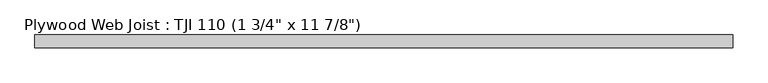
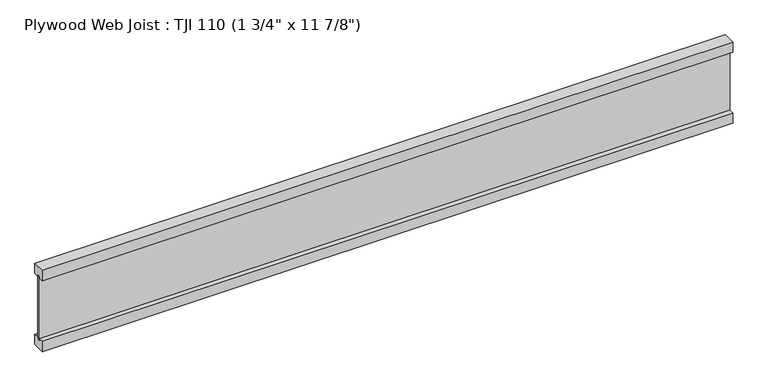
"""IFC4 building model written with IfcOpenShell, lengths in millimetres: beam geometry."""

from ifc_helpers import new_model, si_unit, frame, origin, place, context, project, spatial, polyline, outline, extrude, source, transform, mapped, element, save


def beam_a3ddbb9c(model_context):
    return source(origin(), model_context, "Body", "SweptSolid", [
        extrude(outline(polyline([(-22.225, 150.8125), (22.225, 150.8125), (22.225, 112.7125), (4.7625, 112.7125), (4.7625, 119.0625), (-4.7625, 119.0625), (-4.7625, 112.7125), (-22.225, 112.7125), (-22.225, 150.8125)])), frame((-1236.6625, 0.0, 0.0), z_axis=(1.0, 0.0, 0.0), x_axis=(0.0, 1.0, 0.0)), (0.0, 0.0, 1.0), 2428.875),
        extrude(outline(polyline([(22.225, -112.7125), (22.225, -150.8125), (-22.225, -150.8125), (-22.225, -112.7125), (-4.7625, -112.7125), (-4.7625, -118.3285374), (4.7625, -118.3285374), (4.7625, -112.7125), (22.225, -112.7125)])), frame((-1236.6625, 0.0, 0.0), z_axis=(1.0, 0.0, 0.0), x_axis=(0.0, 1.0, 0.0)), (0.0, 0.0, 1.0), 2428.875),
        extrude(outline(polyline([(1192.2125, 4.7625), (1192.2125, -4.7625), (-1236.6625, -4.7625), (-1236.6625, 4.7625), (1192.2125, 4.7625)])), frame((0.0, 0.0, -118.3285374), z_axis=(0.0, 0.0, 1.0), x_axis=(1.0, 0.0, 0.0)), (0.0, 0.0, 1.0), 237.3910374),
    ])


if __name__ == "__main__":
    model = new_model("IFC4")
    model_context = context("Model", 3, world=origin())
    ifc_project = project(units=[si_unit("LENGTHUNIT", "METRE", prefix="MILLI")], contexts=[model_context])
    site = spatial("IfcSite", under=ifc_project)
    building = spatial("IfcBuilding", under=site)
    placement = place(None, origin())
    beam_shape = beam_a3ddbb9c(model_context)
    element("IfcBeam", 1, ObjectType="Plywood Web Joist : TJI 110 (1 3/4\" x 11 7/8\")", at=placement, inside=building, context=model_context, shape_type="MappedRepresentation", body=[
        mapped(beam_shape, transform((0.0, 0.0, 0.0), x_axis=(1.0, 0.0, 0.0), y_axis=(0.0, 1.0, 0.0), z_axis=(0.0, 0.0, 1.0))),
    ])
    save(model, "model.ifc")

# Revit data of these elements
# Type "Plywood Web Joist : TJI 110 (1 3/4\" x 11 7/8\")"
#   Assembly Code = "B10"
#   Length [instance default] = 5' - 0"
#   b = 0' - 1 3/4"
#   d = 0' - 11 7/8"
#   Structural Material [instance default] = Softwood, Lumber
# Element 1 (IfcBeam, "Plywood Web Joist : TJI 110 (1 3/4\" x 11 7/8\")")
#   Materials on its faces: "Softwood, Lumber"
# Materials
#   "Softwood, Lumber": class "Wood", colour RGB 144 113 62, transparency 0, Description = "Pinus Echinata", Cost = 0
